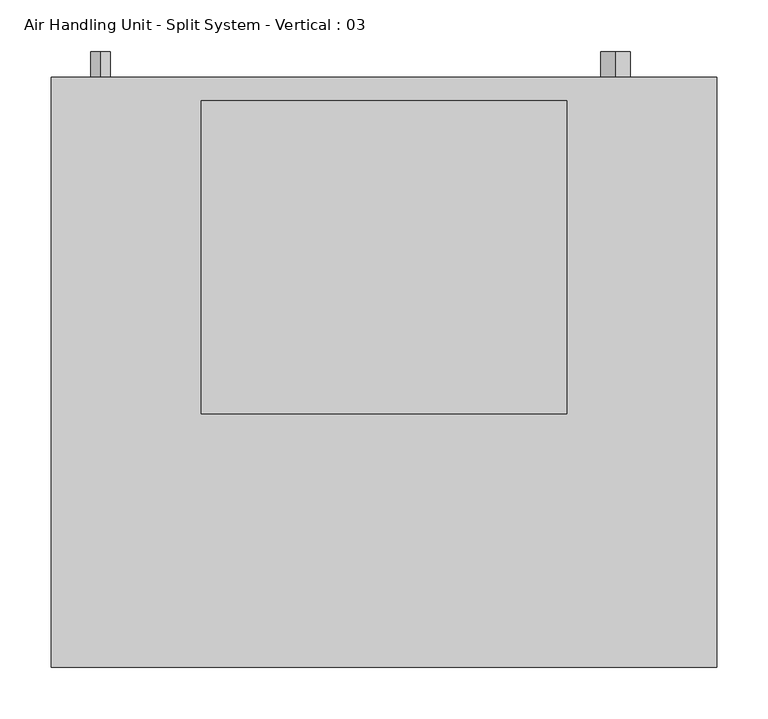
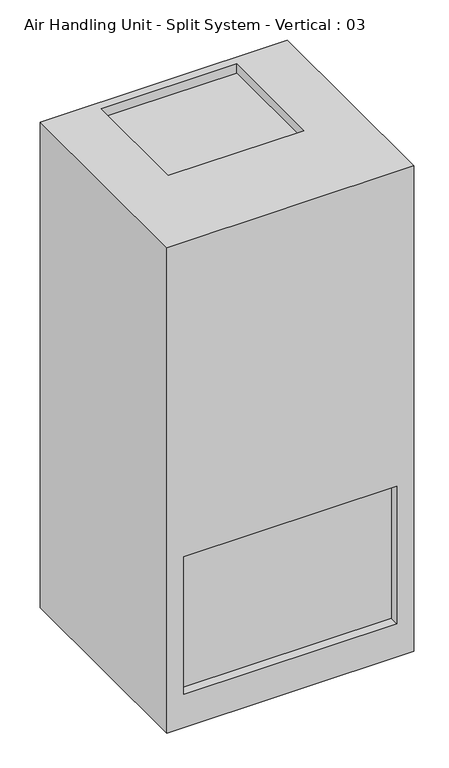
"""IFC4 building model written with IfcOpenShell, lengths in millimetres: proxy geometry, Air Handling Unit - Split System - Vertical : 03."""

import ifcopenshell
import ifcopenshell.guid

model = None  # the IFC model being written
_history = None  # IfcOwnerHistory: only IFC2X3 demands one
_inside = {}  # id of a spatial element -> (the spatial element, [elements in it])
_under = {}  # id of a project, library or spatial element -> (it, [spatial elements below it])
_declared = {}  # id of a project -> (the project, [libraries it declares])
_typed = {}  # id of a type object -> (the type object, [elements of that type])
_made_of = {}  # id of a material, layer set ... -> (it, [elements and type objects made of it])


def new_model(schema):
    """Start an empty IFC model of exactly this schema.

    Asked for "IFC4X3", IfcOpenShell would pick the latest addendum, in which some entities
    have other attributes; the version numbers below select the first issue.
    IFC2X3 requires an IfcOwnerHistory on every rooted entity: one is made here for all.
    """
    global model, _history
    if schema == "IFC4X3":
        model = ifcopenshell.file(schema_version=(4, 3, 0, 0))
    else:
        model = ifcopenshell.file(schema=schema)
    _inside.clear()
    _under.clear()
    _declared.clear()
    _typed.clear()
    _made_of.clear()
    _history = None
    if model.schema == "IFC2X3":
        org = make("IfcOrganization", Name="unknown")
        user = make(
            "IfcPersonAndOrganization",
            ThePerson=make("IfcPerson", FamilyName="unknown"),
            TheOrganization=org,
        )
        app = make(
            "IfcApplication",
            ApplicationDeveloper=org,
            Version="unknown",
            ApplicationFullName="unknown",
            ApplicationIdentifier="unknown",
        )
        _history = make(
            "IfcOwnerHistory",
            OwningUser=user,
            OwningApplication=app,
            ChangeAction="ADDED",
            CreationDate=0,
        )
    return model


def make(cls, **values):
    """One entity of the class cls with the attributes given. An attribute that is None is left unset."""
    return model.create_entity(
        cls, **{name: value for name, value in values.items() if value is not None}
    )


def rooted(cls, **values):
    """An entity with a GlobalId (a new one), such as an element, a storey or a relation."""
    return make(cls, GlobalId=ifcopenshell.guid.new(), OwnerHistory=_history, **values)


def si_unit(unit_type, name, prefix=None):
    """IfcSIUnit, for example si_unit("LENGTHUNIT", "METRE", prefix="MILLI")."""
    return make("IfcSIUnit", UnitType=unit_type, Prefix=prefix, Name=name)


def assignment(units):
    """IfcUnitAssignment: the units of a project."""
    return None if units is None else make("IfcUnitAssignment", Units=units)


def point(xyz):
    """IfcCartesianPoint."""
    return None if xyz is None else make("IfcCartesianPoint", Coordinates=xyz)


def direction(xyz):
    """IfcDirection."""
    return None if xyz is None else make("IfcDirection", DirectionRatios=xyz)


def frame(location, z_axis=None, x_axis=None):
    """IfcAxis2Placement3D, a coordinate frame: its origin and axes. An axis left out is left unset."""
    return make(
        "IfcAxis2Placement3D",
        Location=point(location),
        Axis=direction(z_axis),
        RefDirection=direction(x_axis),
    )


def frame_2d(location, x_axis=None):
    """IfcAxis2Placement2D, a coordinate frame in the plane: its origin and x axis."""
    return make(
        "IfcAxis2Placement2D", Location=point(location), RefDirection=direction(x_axis)
    )


def origin():
    """The frame at (0, 0, 0) with its axes left unset."""
    return frame((0.0, 0.0, 0.0))


def place(relative_to, where):
    """IfcLocalPlacement: puts the frame where relative to a parent placement (None: the world)."""
    return make(
        "IfcLocalPlacement", PlacementRelTo=relative_to, RelativePlacement=where
    )


def context(
    kind, dimensions, precision=None, world=None, true_north=None, identifier=None
):
    """IfcGeometricRepresentationContext, for example the 3D "Model" context."""
    return make(
        "IfcGeometricRepresentationContext",
        ContextIdentifier=identifier,
        ContextType=kind,
        CoordinateSpaceDimension=dimensions,
        Precision=precision,
        WorldCoordinateSystem=world,
        TrueNorth=true_north,
    )


def project(units=None, contexts=None):
    """IfcProject with its units and contexts."""
    return rooted(
        "IfcProject",
        Name="project",
        RepresentationContexts=contexts,
        UnitsInContext=assignment(units),
    )


def spatial(cls, under=None, at=None, **own):
    """A site, building, storey or space (cls), placed at a placement, below another one or the project."""
    s = rooted(cls, ObjectPlacement=at, **own)
    if under is not None:
        _under.setdefault(under.id(), (under, []))[1].append(s)
    return s


def circle_curve(where, radius):
    """IfcCircle in the frame where."""
    return make("IfcCircle", Position=where, Radius=radius)


def trimmed(basis, trim1, trim2, sense, master):
    """IfcTrimmedCurve: the piece of a basis curve between two trims."""
    return make(
        "IfcTrimmedCurve",
        BasisCurve=basis,
        Trim1=trim1,
        Trim2=trim2,
        SenseAgreement=sense,
        MasterRepresentation=master,
    )


def segment(curve, same_sense, transition):
    """IfcCompositeCurveSegment."""
    return make(
        "IfcCompositeCurveSegment",
        Transition=transition,
        SameSense=same_sense,
        ParentCurve=curve,
    )


def composite_curve(segments, self_intersect=None):
    """IfcCompositeCurve: segments joined end to end."""
    return make("IfcCompositeCurve", Segments=segments, SelfIntersect=self_intersect)


def outline(outer, holes=None, kind="AREA"):
    """IfcArbitraryClosedProfileDef: a profile drawn as a closed curve; with holes, ...WithVoids."""
    if holes is None:
        return make("IfcArbitraryClosedProfileDef", ProfileType=kind, OuterCurve=outer)
    return make(
        "IfcArbitraryProfileDefWithVoids",
        ProfileType=kind,
        OuterCurve=outer,
        InnerCurves=holes,
    )


def extrude(swept, where, along, depth):
    """IfcExtrudedAreaSolid: the profile swept, set in the frame where, extruded along a direction by depth."""
    return make(
        "IfcExtrudedAreaSolid",
        SweptArea=swept,
        Position=where,
        ExtrudedDirection=direction(along),
        Depth=depth,
    )


def faces_of(points, faces, orient=None, outer=None):
    """IfcFace entities. A face is a list of loops; a loop is a list of indices into points, from 0.

    orient and outer hold one flag for each loop. By default every Orientation is true, the
    first loop of a face is its IfcFaceOuterBound and the others are IfcFaceBound.
    """
    made = []
    for i, loops in enumerate(faces):
        bounds = []
        for j, loop in enumerate(loops):
            is_outer = j == 0 if outer is None else outer[i][j]
            bounds.append(
                make(
                    "IfcFaceOuterBound" if is_outer else "IfcFaceBound",
                    Bound=make("IfcPolyLoop", Polygon=[points[k] for k in loop]),
                    Orientation=True if orient is None else orient[i][j],
                )
            )
        made.append(make("IfcFace", Bounds=bounds))
    return made


def faceted_brep(points, faces, orient=None, outer=None, voids=None):
    """IfcFacetedBrep: a solid bounded by flat faces; with voids (closed shells), ...WithVoids."""
    shared = [point(p) for p in points]
    hull = make("IfcClosedShell", CfsFaces=faces_of(shared, faces, orient, outer))
    if voids is None:
        return make("IfcFacetedBrep", Outer=hull)
    return make(
        "IfcFacetedBrepWithVoids",
        Outer=hull,
        Voids=[
            make(cls, CfsFaces=faces_of(shared, fs, o, b)) for cls, fs, o, b in voids
        ],
    )


def shape(context_of_items, identifier, shape_type, items):
    """IfcShapeRepresentation: the items that make up one representation, for example the "Body"."""
    return make(
        "IfcShapeRepresentation",
        ContextOfItems=context_of_items,
        RepresentationIdentifier=identifier,
        RepresentationType=shape_type,
        Items=items,
    )


def source(mapping_origin, context_of_items, identifier, shape_type, items):
    """IfcRepresentationMap: a shape defined once, which mapped items show again and again."""
    return make(
        "IfcRepresentationMap",
        MappingOrigin=mapping_origin,
        MappedRepresentation=shape(context_of_items, identifier, shape_type, items),
    )


def transform(
    local_origin,
    x_axis=None,
    y_axis=None,
    z_axis=None,
    scale=None,
    scale2=None,
    scale3=None,
    uniform=True,
):
    """IfcCartesianTransformationOperator3D, or its non-uniform kind. x_axis, y_axis, z_axis: its Axis1, 2, 3."""
    if uniform:
        return make(
            "IfcCartesianTransformationOperator3D",
            Axis1=direction(x_axis),
            Axis2=direction(y_axis),
            LocalOrigin=point(local_origin),
            Scale=scale,
            Axis3=direction(z_axis),
        )
    return make(
        "IfcCartesianTransformationOperator3DnonUniform",
        Axis1=direction(x_axis),
        Axis2=direction(y_axis),
        LocalOrigin=point(local_origin),
        Scale=scale,
        Axis3=direction(z_axis),
        Scale2=scale2,
        Scale3=scale3,
    )


def mapped(mapping_source, mapping_target):
    """IfcMappedItem: shows the shape of a source again, moved by a transform."""
    return make(
        "IfcMappedItem", MappingSource=mapping_source, MappingTarget=mapping_target
    )


def made_of(thing, what):
    """Note that an element or type object is made of a material, layer set ...; save() writes the relation."""
    if what is not None:
        _made_of.setdefault(what.id(), (what, []))[1].append(thing)
    return thing


def element(
    cls,
    number,
    at=None,
    inside=None,
    cuts=None,
    type_object=None,
    material=None,
    context=None,
    identifier="Body",
    shape_type=None,
    held_by="IfcProductDefinitionShape",
    body=None,
    shapes=None,
    **own,
):
    """One element of the class cls, such as IfcWall. Its Tag is "e" and its number.

    at: its placement. inside: the storey or other place that contains it. cuts: it is an
    opening in that element (IfcRelVoidsElement). A single representation is given by context,
    identifier, shape_type and body (its items); several are given by shapes. held_by: the class
    of the entity that holds the representations. save() writes the other relations.
    """
    e = rooted(cls, Tag="e%d" % number, ObjectPlacement=at, **own)
    if body is not None:
        shapes = [shape(context, identifier, shape_type, body)]
    if shapes is not None:
        e.Representation = make(held_by, Representations=shapes)
    if inside is not None:
        _inside.setdefault(inside.id(), (inside, []))[1].append(e)
    if cuts is not None:
        rooted(
            "IfcRelVoidsElement", RelatingBuildingElement=cuts, RelatedOpeningElement=e
        )
    if type_object is not None:
        _typed.setdefault(type_object.id(), (type_object, []))[1].append(e)
    return made_of(e, material)


def aggregate(whole, parts):
    """IfcRelAggregates: a whole, such as a stair, and the parts it consists of."""
    return rooted("IfcRelAggregates", RelatingObject=whole, RelatedObjects=parts)


def save(model, path):
    """Write the relations noted so far, then the file.

    IfcRelAggregates (storeys below a building ...), IfcRelContainedInSpatialStructure (elements
    in a storey), IfcRelDefinesByType, IfcRelAssociatesMaterial and IfcRelDeclares: one each for
    every whole, place, type object, material and project.
    """
    for whole, parts in _under.values():
        aggregate(whole, parts)
    for where, things in _inside.values():
        rooted(
            "IfcRelContainedInSpatialStructure",
            RelatedElements=things,
            RelatingStructure=where,
        )
    for kind, things in _typed.values():
        rooted("IfcRelDefinesByType", RelatedObjects=things, RelatingType=kind)
    for what, things in _made_of.values():
        rooted("IfcRelAssociatesMaterial", RelatedObjects=things, RelatingMaterial=what)
    for by, libraries in _declared.values():
        rooted("IfcRelDeclares", RelatingContext=by, RelatedDefinitions=libraries)
    model.write(path)


def air_handling_unit_split_system_vertical_03_658e3e83(model_context):
    return source(origin(), model_context, "Body", "SolidModel", [
        extrude(outline(composite_curve([segment(trimmed(circle_curve(frame_2d((132.55625, -275.828125)), 9.525), [point((142.08125, -275.828125))], [point((123.03125, -275.828125))], False, "CARTESIAN"), True, "CONTINUOUS"), segment(trimmed(circle_curve(frame_2d((132.55625, -275.828125)), 9.525), [point((123.03125, -275.828125))], [point((142.08125, -275.828125))], False, "CARTESIAN"), True, "CONTINUOUS")], self_intersect=False)), frame((0.0, 287.0398438, 0.0), z_axis=(0.0, 1.0, 0.0), x_axis=(0.0, 0.0, 1.0)), (0.0, 0.0, 1.0), 25.4),
        extrude(outline(composite_curve([segment(trimmed(circle_curve(frame_2d((394.096875, 225.425)), 4.7625), [point((398.859375, 225.425))], [point((389.334375, 225.425))], False, "CARTESIAN"), True, "CONTINUOUS"), segment(trimmed(circle_curve(frame_2d((394.096875, 225.425)), 4.7625), [point((389.334375, 225.425))], [point((398.859375, 225.425))], False, "CARTESIAN"), True, "CONTINUOUS")], self_intersect=False)), frame((0.0, 287.0398438, 0.0), z_axis=(0.0, 1.0, 0.0), x_axis=(0.0, 0.0, 1.0)), (0.0, 0.0, 1.0), 25.4),
        extrude(outline(composite_curve([segment(trimmed(circle_curve(frame_2d((465.534375, 225.425)), 14.2875), [point((479.821875, 225.425))], [point((451.246875, 225.425))], False, "CARTESIAN"), True, "CONTINUOUS"), segment(trimmed(circle_curve(frame_2d((465.534375, 225.425)), 14.2875), [point((451.246875, 225.425))], [point((479.821875, 225.425))], False, "CARTESIAN"), True, "CONTINUOUS")], self_intersect=False)), frame((0.0, 287.0398438, 0.0), z_axis=(0.0, 1.0, 0.0), x_axis=(0.0, 0.0, 1.0)), (0.0, 0.0, 1.0), 25.4),
        faceted_brep([(323.85, 287.0398438, 1346.2), (-323.85, 287.0398438, 1346.2), (-323.85, -287.0398438, 1346.2), (323.85, -287.0398438, 1346.2), (177.8, 264.2195313, 1346.2), (177.8, -40.5804687, 1346.2), (-177.8, -40.5804687, 1346.2), (-177.8, 264.2195313, 1346.2), (323.85, 287.0398438, 0.0), (323.85, -287.0398438, 0.0), (-323.85, -287.0398438, 0.0), (-323.85, 287.0398438, 0.0), (279.4, -287.0398438, 472.8765625), (279.4, -287.0398438, 91.8765625), (-279.4, -287.0398438, 91.8765625), (-279.4, -287.0398438, 472.8765625), (177.8, 264.2195313, 1320.8), (-177.8, 264.2195313, 1320.8), (-177.8, -40.5804687, 1320.8), (177.8, -40.5804687, 1320.8), (279.4, -261.6398438, 472.8765625), (-279.4, -261.6398438, 472.8765625), (-279.4, -261.6398438, 91.8765625), (279.4, -261.6398438, 91.8765625)], [[[0, 1, 2, 3], [4, 5, 6, 7]], [[8, 9, 10, 11]], [[1, 0, 8, 11]], [[2, 1, 11, 10]], [[3, 2, 10, 9], [12, 13, 14, 15]], [[0, 3, 9, 8]], [[16, 17, 18, 19]], [[16, 19, 5, 4]], [[19, 18, 6, 5]], [[18, 17, 7, 6]], [[17, 16, 4, 7]], [[20, 21, 22, 23]], [[20, 23, 13, 12]], [[23, 22, 14, 13]], [[22, 21, 15, 14]], [[21, 20, 12, 15]]]),
    ])


if __name__ == "__main__":
    model = new_model("IFC4")
    model_context = context("Model", 3, world=origin())
    ifc_project = project(units=[si_unit("LENGTHUNIT", "METRE", prefix="MILLI")], contexts=[model_context])
    site = spatial("IfcSite", under=ifc_project)
    building = spatial("IfcBuilding", under=site)
    placement = place(None, origin())
    air_handling_unit_split_system_vertical_03_shape = air_handling_unit_split_system_vertical_03_658e3e83(model_context)
    element("IfcBuildingElementProxy", 1, Name="Air Handling Unit - Split System - Vertical : 03", ObjectType="Air Handling Unit - Split System - Vertical : 03", at=placement, inside=building, context=model_context, shape_type="MappedRepresentation", body=[
        mapped(air_handling_unit_split_system_vertical_03_shape, transform((0.0, 0.0, 0.0), x_axis=(1.0, 0.0, 0.0), y_axis=(0.0, 1.0, 0.0), z_axis=(0.0, 0.0, 1.0))),
    ])
    save(model, "model.ifc")

# Revit data of these elements
# Project information
#   Project Issue Date = "Issue Date"
#   Project Status = "Project Status"
#   Client Name = "Owner"
#   Project Address = "Enter address here"
#   Project Name = "Project Name"
#   Project Number = "Project Number"
# Type "Air Handling Unit - Split System - Vertical : 03"
#   PartShape = "Rectangular Duct"
#   Model = "03"
#   Voltage = 208 V
#   UnitWidth = 2' - 1 1/2"
#   UnitHeight = 4' - 5"
#   UnitDepth = 1' - 10 77/128"
#   Width1 = 1' - 2"
#   SupplyOpeningOffset = 0' - 0 115/128"
#   Outlet Radius = 9/16"
#   Outlet Diameter = 1 1/8"
#   Inlet Radius = 3/16"
#   Inlet Diameter = 3/8"
#   Height1 = 1' - 0"
#   SupplyConnectorOffset = 0' - 6"
#   Width2 = 1' - 10"
#   Height2 = 1' - 3"
#   ReturnConnectorOffset = 0' - 7 1/2"
#   ReturnAirOffset = 0' - 3 79/128"
#   Half UnitWidth = 1' - 0 3/4"
#   Drain Flow [instance default] = 0 GPM
#   C3 Offset 1 = 1' - 6 21/64"
#   Apparent Load = 10816 VA
#   External Static Pressure [instance default] = 0.50 in-wg
#   Air Flow [instance default] = 1170 CFM
#   Number of Poles = 3
#   Load Classification = Cooling
#   Default Elevation = 0
#   Assembly Code = ""
